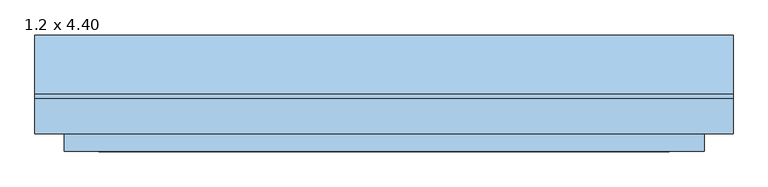
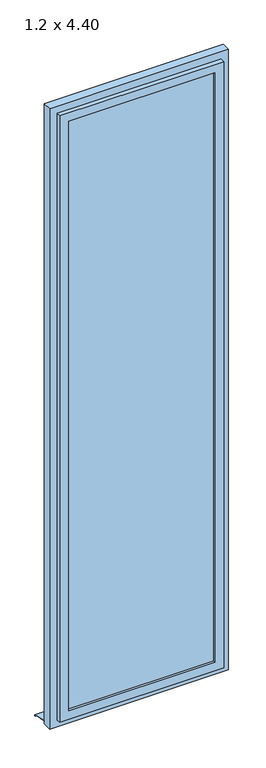
"""IFC4 building model written with IfcOpenShell, lengths in millimetres: window geometry, Fenstertür 1-flg : 1.2 x 4.40."""

from ifc_helpers import new_model, si_unit, frame, origin, place, context, project, spatial, polyline, outline, extrude, faceted_brep, source, transform, mapped, element, save


def window_1_2_x_4_40_23940e03(model_context):
    return source(origin(), model_context, "Body", "SolidModel", [
        extrude(outline(polyline([(4400.0, 600.0), (4400.0, -600.0), (0.0, -600.0), (0.0, 600.0), (4400.0, 600.0)]), holes=[polyline([(4320.0, 520.0), (80.0, 520.0), (80.0, -520.0), (4320.0, -520.0), (4320.0, 520.0)])]), frame((0.0, 10.0, 0.0), z_axis=(0.0, 1.0, 0.0), x_axis=(0.0, 0.0, 1.0)), (0.0, 0.0, 1.0), 60.0),
        faceted_brep([(550.0, 10.0, 4350.0), (550.0, -20.0, 4350.0), (550.0, -20.0, 50.0), (550.0, 10.0, 50.0), (-550.0, -20.0, 4350.0), (-550.0, -20.0, 50.0), (490.0, -20.0, 110.0), (-490.0, -20.0, 110.0), (-490.0, -20.0, 4290.0), (490.0, -20.0, 4290.0), (-550.0, 10.0, 50.0), (-550.0, 10.0, 4350.0), (520.0, 10.0, 4320.0), (-520.0, 10.0, 4320.0), (-520.0, 10.0, 80.0), (520.0, 10.0, 80.0), (520.0, 40.0, 4320.0), (520.0, 40.0, 80.0), (-520.0, 40.0, 80.0), (-520.0, 40.0, 4320.0), (490.0, 40.0, 4290.0), (-490.0, 40.0, 4290.0), (-490.0, 40.0, 110.0), (490.0, 40.0, 110.0)], [[[0, 1, 2, 3]], [[1, 4, 5, 2], [6, 7, 8, 9]], [[3, 2, 5, 10]], [[3, 10, 11, 0], [12, 13, 14, 15]], [[16, 12, 15, 17]], [[17, 15, 14, 18]], [[17, 18, 19, 16], [20, 21, 22, 23]], [[9, 20, 23, 6]], [[6, 23, 22, 7]], [[10, 5, 4, 11]], [[18, 14, 13, 19]], [[7, 22, 21, 8]], [[11, 4, 1, 0]], [[19, 13, 12, 16]], [[8, 21, 20, 9]]]),
        extrude(outline(polyline([(80.0221543, 20.0), (180.0, 0.0), (180.0, -10.0), (178.0, -10.0), (178.0, -1.6395366), (79.8240723, 18.0), (70.0, 18.0), (70.0, 20.0), (80.0221543, 20.0)])), frame((-600.0, 0.0, 0.0), z_axis=(1.0, 0.0, 0.0), x_axis=(0.0, 1.0, 0.0)), (0.0, 0.0, 1.0), 1200.0),
        extrude(outline(polyline([(490.0, -5.0), (-490.0, -5.0), (-490.0, 25.0), (490.0, 25.0), (490.0, -5.0)])), frame((0.0, 0.0, 110.0), z_axis=(0.0, 0.0, 1.0), x_axis=(1.0, 0.0, 0.0)), (0.0, 0.0, 1.0), 4180.0),
    ])


if __name__ == "__main__":
    model = new_model("IFC4")
    model_context = context("Model", 3, world=origin())
    ifc_project = project(units=[si_unit("LENGTHUNIT", "METRE", prefix="MILLI")], contexts=[model_context])
    site = spatial("IfcSite", under=ifc_project)
    building = spatial("IfcBuilding", under=site)
    placement = place(None, origin())
    window_1_2_x_4_40_shape = window_1_2_x_4_40_23940e03(model_context)
    element("IfcWindow", 1, ObjectType="Fenstertür 1-flg : 1.2 x 4.40", at=placement, inside=building, context=model_context, shape_type="MappedRepresentation", body=[
        mapped(window_1_2_x_4_40_shape, transform((0.0, 0.0, 0.0), x_axis=(1.0, 0.0, 0.0), y_axis=(0.0, 1.0, 0.0), z_axis=(0.0, 0.0, 1.0))),
    ])
    save(model, "model.ifc")

# Revit data of these elements
# Type "Fenstertür 1-flg : 1.2 x 4.40"
#   Type Mark = "56"
#   Operation = "SinglePanel"
#   Construction Type Id = "GSP4R"
#   Keynote = "16.05.01"
#   Analytic Construction = "1/8 Zoll Pilkington-Verglasung einfach"
#   Visual Light Transmittance = 0.9
#   Thermal Resistance (R) = 0.1491 (m²·K)/W
#   Solar Heat Gain Coefficient = 0.86
#   Rough Width = 1.200 m
#   Rough Height = 4.400 m
#   Heat Transfer Coefficient (U) = 6.7069 W/(m²·K)
#   Rahmentiefe = 0.060 m
#   Rahmenhöhe - unten = 0.080 m
#   Rahmenhöhe - oben = 0.080 m
#   Rahmenbreite = 0.080 m
#   Height = 4.400 m
#   Tiefe Flügel = 0.060 m
#   Flügelbreite = 0.060 m
#   Einbautiefe (von außen) [instance default] = 0.080 m
#   Width = 1.200 m
#   Kippflügel [instance default] = yes
#   Drehflügel im Grundriss darstellen [instance default] = yes
#   Drehflügel 1 [instance default] = yes
#   Rahmen 1 [instance default] = none
#   Glas [instance default] = none
#   Flügel [instance default] = none
#   Fensterbank Außenseite [instance default] = none
#   Wall Closure = (empty or 0)
# Element 1 (IfcWindow, "Fenstertür 1-flg : 1.2 x 4.40")
#   Materials on its faces: "Kunststoff - Weiß", "Glas"
# Materials
#   "Kunststoff - Weiß": class "Kunststoff", colour RGB 249 249 249, transparency 0, Cost = 0
#   "Glas": class "Glas", colour RGB 0 0 255, transparency 0.75, Comments = "Render-Darstellung nicht aktualisiert ", Cost = 0
